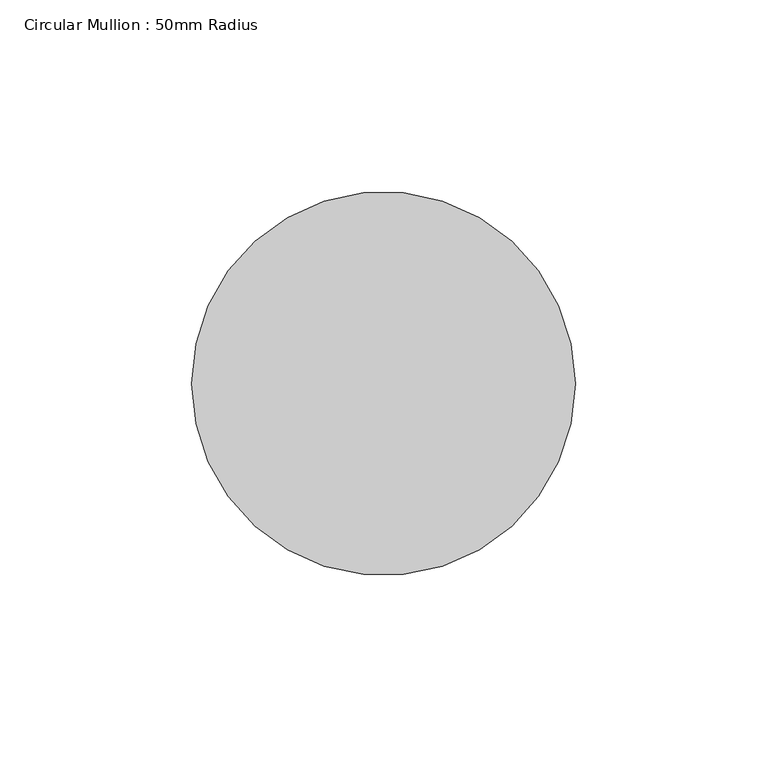
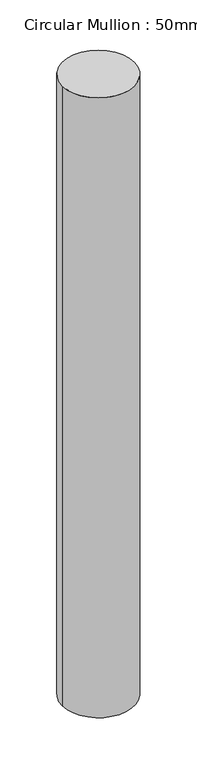
"""IFC4 building model written with IfcOpenShell, lengths in millimetres: member geometry, Circular Mullion : 50mm Radius."""

from ifc_helpers import new_model, si_unit, point, frame, origin, origin_2d, place, context, project, spatial, circle_curve, trimmed, segment, composite_curve, outline, extrude, source, transform, mapped, element, save


def circular_mullion_50mm_radius_ed60fe0e(model_context):
    return source(origin(), model_context, "Body", "SweptSolid", [
        extrude(outline(composite_curve([segment(trimmed(circle_curve(origin_2d(), 50.0), [point((50.0, 0.0))], [point((-50.0, 0.0))], False, "CARTESIAN"), True, "CONTINUOUS"), segment(trimmed(circle_curve(origin_2d(), 50.0), [point((-50.0, 0.0))], [point((50.0, 0.0))], False, "CARTESIAN"), True, "CONTINUOUS")], self_intersect=False)), frame((0.0, 0.0, -910.1663352), z_axis=(0.0, 0.0, 1.0), x_axis=(1.0, 0.0, 0.0)), (0.0, 0.0, 1.0), 910.1663352),
    ])


if __name__ == "__main__":
    model = new_model("IFC4")
    model_context = context("Model", 3, world=origin())
    ifc_project = project(units=[si_unit("LENGTHUNIT", "METRE", prefix="MILLI")], contexts=[model_context])
    site = spatial("IfcSite", under=ifc_project)
    building = spatial("IfcBuilding", under=site)
    placement = place(None, origin())
    circular_mullion_50mm_radius_shape = circular_mullion_50mm_radius_ed60fe0e(model_context)
    element("IfcMember", 1, ObjectType="Circular Mullion : 50mm Radius", at=placement, inside=building, context=model_context, shape_type="MappedRepresentation", body=[
        mapped(circular_mullion_50mm_radius_shape, transform((0.0, 0.0, 0.0), x_axis=(1.0, 0.0, 0.0), y_axis=(0.0, 1.0, 0.0), z_axis=(0.0, 0.0, 1.0))),
    ])
    save(model, "model.ifc")

# Revit data of these elements
# Type "Circular Mullion : 50mm Radius"
#   built-in parameter 1007350 = 0.164042 (stored number, unit not read)
# Element 1 (IfcMember, "Circular Mullion : 50mm Radius")
#   Materials on its faces: "Aluminium"
# Materials
#   "Aluminium": class "Metal", colour RGB 247 247 247, transparency 0, Description = "Aluminium 6061", Cost = 0
